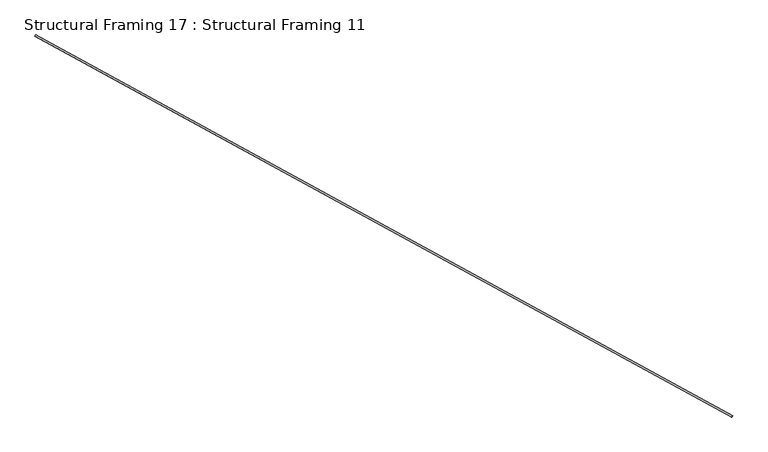
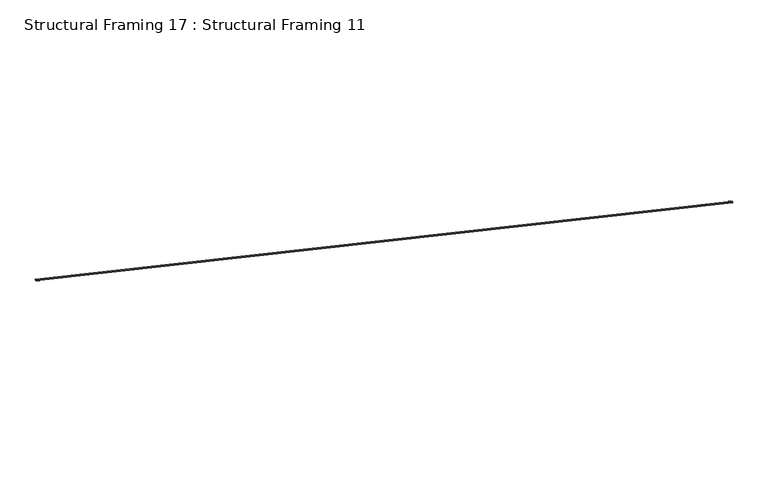
"""IFC4 building model written with IfcOpenShell, lengths in millimetres: beam geometry, Structural Framing 17 : Structural Framing 11."""

from ifc_helpers import new_model, si_unit, point, frame, origin, origin_2d, place, context, project, spatial, circle_curve, trimmed, segment, composite_curve, outline, extrude, source, transform, mapped, element, save


def structural_framing_17_structural_framing_11_a142ccf5(model_context):
    return source(origin(), model_context, "Body", "SweptSolid", [
        extrude(outline(composite_curve([segment(trimmed(circle_curve(origin_2d(), 6.35), [point((0.0, -6.35))], [point((0.0, 6.3499999))], False, "CARTESIAN"), True, "CONTINUOUS"), segment(trimmed(circle_curve(origin_2d(), 6.35), [point((0.0, 6.3499999))], [point((0.0, -6.35))], False, "CARTESIAN"), True, "CONTINUOUS")], self_intersect=False)), frame((12605.5334333, 10048.6776702, 4933.3856456), z_axis=(0.8714985593718692, -0.4757560037149618, 0.11893900092873713), x_axis=(0.0, 0.24253562503632653, 0.9701425001453335)), (0.0, 0.0, 1.0), 6120.4961437),
    ])


if __name__ == "__main__":
    model = new_model("IFC4")
    model_context = context("Model", 3, world=origin())
    ifc_project = project(units=[si_unit("LENGTHUNIT", "METRE", prefix="MILLI")], contexts=[model_context])
    site = spatial("IfcSite", under=ifc_project)
    building = spatial("IfcBuilding", under=site)
    placement = place(None, origin())
    structural_framing_17_structural_framing_11_shape = structural_framing_17_structural_framing_11_a142ccf5(model_context)
    element("IfcBeam", 1, ObjectType="Structural Framing 17 : Structural Framing 11", at=placement, inside=building, context=model_context, shape_type="MappedRepresentation", body=[
        mapped(structural_framing_17_structural_framing_11_shape, transform((0.0, 0.0, 0.0), x_axis=(1.0, 0.0, 0.0), y_axis=(0.0, 1.0, 0.0), z_axis=(0.0, 0.0, 1.0))),
    ])
    save(model, "model.ifc")

# Revit data of these elements
# Type "Structural Framing 17 : Structural Framing 11"
#   Structural Material [instance default] = EXISTING LATERAL BRACING (1/4" CABLE)
# Element 1 (IfcBeam, "Structural Framing 17 : Structural Framing 11")
#   Materials on its faces: "EXISTING LATERAL BRACING (1/4\" CABLE)"
# Materials
#   "EXISTING LATERAL BRACING (1/4\" CABLE)": class "Generic", colour RGB 120 120 120, transparency 0, Cost = 0
